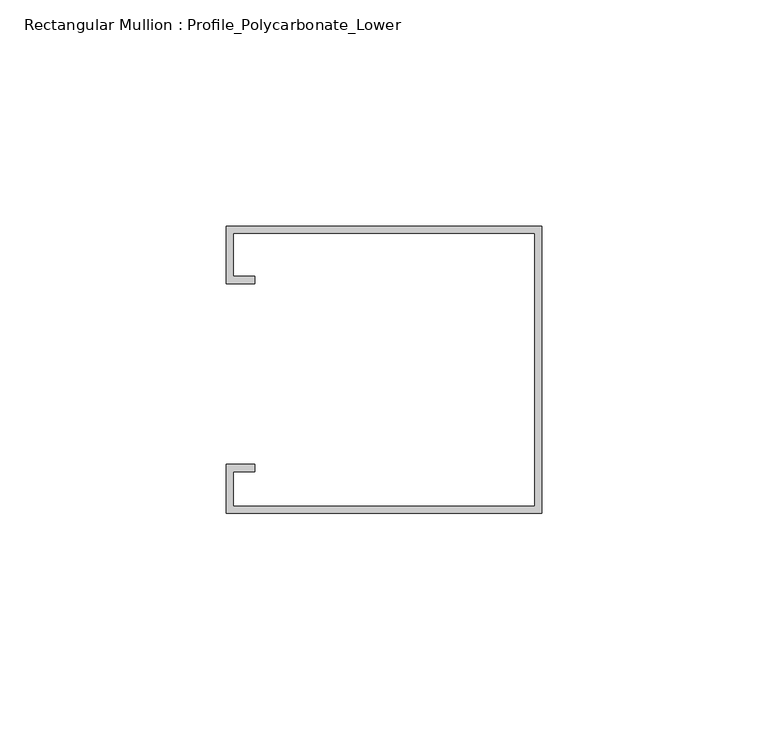
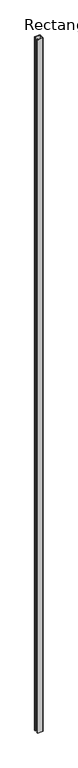
"""IFC4 building model written with IfcOpenShell, lengths in millimetres: member geometry, Rectangular Mullion : Profile_Polycarbonate_Lower."""

from ifc_helpers import new_model, si_unit, frame, origin, place, context, project, spatial, polyline, outline, extrude, source, transform, mapped, element, save


def rectangular_mullion_profile_polycarbonate_lower_bae52e08(model_context):
    return source(origin(), model_context, "Body", "SweptSolid", [
        extrude(outline(polyline([(0.0, 32.7), (0.0, -30.8), (-69.85, -30.8), (-69.85, -20.0), (-63.5, -20.0), (-63.5, -21.5875), (-68.2625, -21.5875), (-68.2625, -29.2125), (-1.5875, -29.2125), (-1.5875, 31.1125), (-68.2625, 31.1125), (-68.2625, 21.5875), (-63.5, 21.5875), (-63.5, 20.0), (-69.85, 20.0), (-69.85, 32.7), (0.0, 32.7)])), frame((0.0, 0.0, -9240.8375), z_axis=(0.0, 0.0, 1.0), x_axis=(1.0, 0.0, 0.0)), (0.0, 0.0, 1.0), 9240.8375),
    ])


if __name__ == "__main__":
    model = new_model("IFC4")
    model_context = context("Model", 3, world=origin())
    ifc_project = project(units=[si_unit("LENGTHUNIT", "METRE", prefix="MILLI")], contexts=[model_context])
    site = spatial("IfcSite", under=ifc_project)
    building = spatial("IfcBuilding", under=site)
    placement = place(None, origin())
    rectangular_mullion_profile_polycarbonate_lower_shape = rectangular_mullion_profile_polycarbonate_lower_bae52e08(model_context)
    element("IfcMember", 1, ObjectType="Rectangular Mullion : Profile_Polycarbonate_Lower", at=placement, inside=building, context=model_context, shape_type="MappedRepresentation", body=[
        mapped(rectangular_mullion_profile_polycarbonate_lower_shape, transform((0.0, 0.0, 0.0), x_axis=(1.0, 0.0, 0.0), y_axis=(0.0, 1.0, 0.0), z_axis=(0.0, 0.0, 1.0))),
    ])
    save(model, "model.ifc")

# Revit data of these elements
# Type "Rectangular Mullion : Profile_Polycarbonate_Lower"
#   built-in parameter 1007322 = 0.208333 (stored number, unit not read)
#   built-in parameter 1007321 = 0 (stored number, unit not read)
#   built-in parameter 1007320 = 0.00520833 (stored number, unit not read)
# Element 1 (IfcMember, "Rectangular Mullion : Profile_Polycarbonate_Lower")
#   Materials on its faces: "ALUMINUM PROFILE AT POLYCARBONATE PANEL"
# Materials
#   "ALUMINUM PROFILE AT POLYCARBONATE PANEL": class "Metal", colour RGB 244 244 244, transparency 0, Description = "Aluminum 6061", Cost = 0
